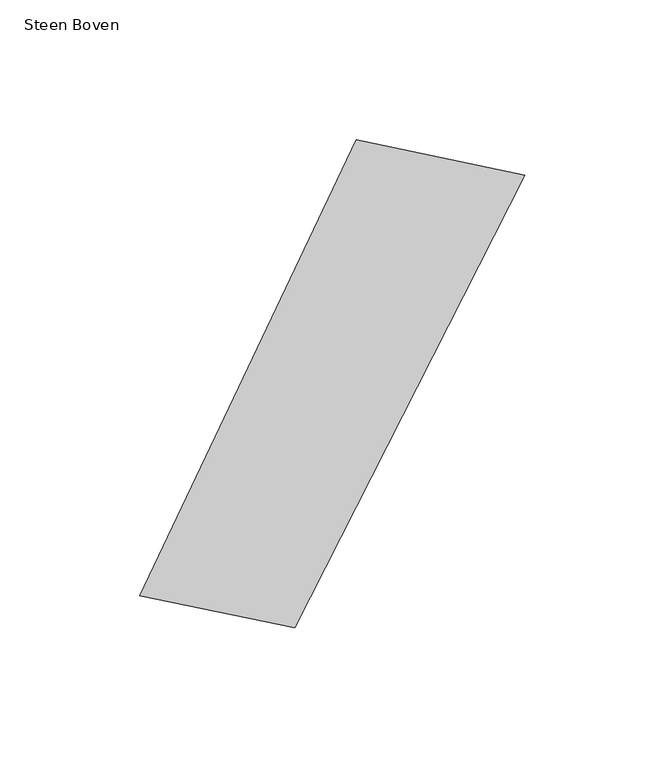
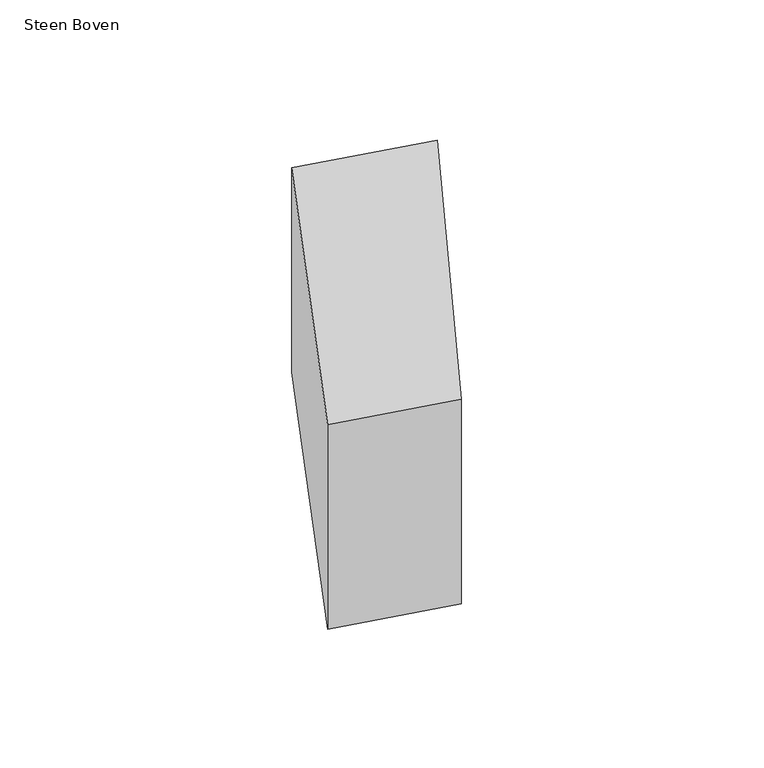
"""IFC4 building model written with IfcOpenShell, lengths in millimetres: proxy geometry, 00_GMA_steen_versie_4 : Steen Boven."""

from ifc_helpers import new_model, si_unit, origin, origin_with_axes, place, context, project, spatial, polyline, outline, extrude, source, transform, mapped, element, save


def steen_boven_110f7231(model_context):
    return source(origin(), model_context, "Body", "SweptSolid", [
        extrude(outline(polyline([(142.9092745, 152.750846), (60.6725408, -9.0611812), (5.4459382, 2.4596603), (82.7689403, 165.2652214), (142.9092745, 152.750846)])), origin_with_axes(), (0.0, 0.0, 1.0), 100.0),
    ])


if __name__ == "__main__":
    model = new_model("IFC4")
    model_context = context("Model", 3, world=origin())
    ifc_project = project(units=[si_unit("LENGTHUNIT", "METRE", prefix="MILLI")], contexts=[model_context])
    site = spatial("IfcSite", under=ifc_project)
    building = spatial("IfcBuilding", under=site)
    placement = place(None, origin())
    steen_boven_shape = steen_boven_110f7231(model_context)
    element("IfcBuildingElementProxy", 1, Name="00_GMA_steen_versie_4 : Steen Boven", ObjectType="00_GMA_steen_versie_4 : Steen Boven", at=placement, inside=building, context=model_context, shape_type="MappedRepresentation", body=[
        mapped(steen_boven_shape, transform((0.0, 0.0, 0.0), x_axis=(1.0, 0.0, 0.0), y_axis=(0.0, 1.0, 0.0), z_axis=(0.0, 0.0, 1.0))),
    ])
    save(model, "model.ifc")

# Revit data of these elements
# Type "00_GMA_steen_versie_4 : Steen Boven"
#   StootVoegHalfBoven [instance default] = 5 mm
#   StootVoegHalf [instance default] = 5 mm
#   StootVoegBreedteOnder = 10 mm
#   StootVoegBreedteBoven = 10 mm
#   Steendikte = 100 mm
#   LintVoegOnderHalf = 5 mm
#   LintVoegOnder = 10 mm
#   LintVoegBovenHalf = 0 mm
#   LintVoegBoven = 0 mm
#   materiaal = none
#   MateriaalVoeg = none
#   Default Elevation = 0
